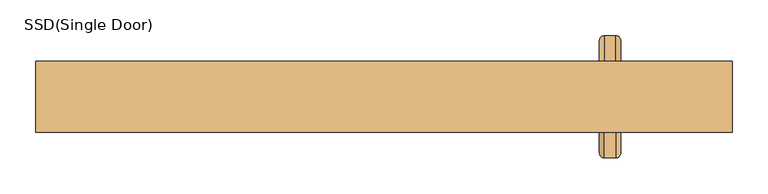
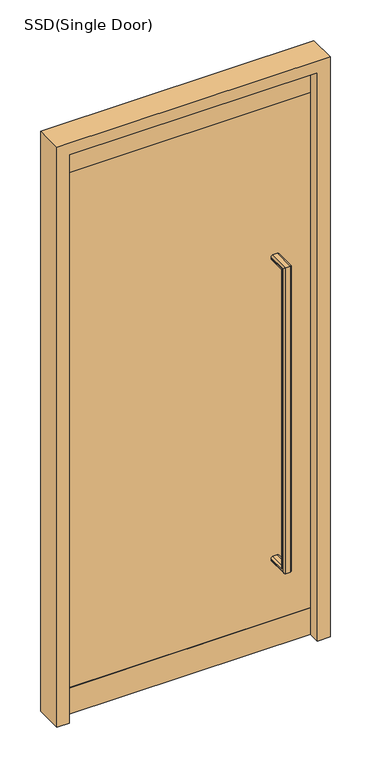
"""IFC4 building model written with IfcOpenShell, lengths in millimetres: door geometry, SSD(Single Door) : H_DR_AR B12_Door_Single_Glass_W1000xH2200_SSD-1."""

from ifc_helpers import new_model, si_unit, frame, origin, origin_with_axes, place, context, project, spatial, polyline, circle_curve, ellipse_curve, outline, extrude, source, transform, mapped, element, save
from ifc_brep_helpers import plane_surface, cylinder_surface, advanced_brep


def ssd_single_door_b9475c77(model_context):
    return source(origin(), model_context, "Body", "SolidModel", [
        extrude(outline(polyline([(0.0, -490.0), (0.0, -445.0), (2155.0, -445.0), (2155.0, 445.0), (0.0, 445.0), (0.0, 490.0), (2200.0, 490.0), (2200.0, -490.0), (0.0, -490.0)])), frame((0.0, -7.0, 0.0), z_axis=(0.0, 1.0, 0.0), x_axis=(0.0, 0.0, 1.0)), (0.0, 0.0, 1.0), 100.0),
        advanced_brep(
        [(310.0, 37.0, 1485.0), (326.0, 37.0, 1485.0), (333.0, 37.0, 1478.0), (333.0, 37.0, 1475.0), (326.0, 37.0, 1468.0), (310.0, 37.0, 1468.0), (303.0, 37.0, 1475.0), (303.0, 37.0, 1478.0), (310.0, 37.0, 325.0), (303.0, 37.0, 332.0), (303.0, 37.0, 335.0), (310.0, 37.0, 342.0), (326.0, 37.0, 342.0), (333.0, 37.0, 335.0), (333.0, 37.0, 332.0), (326.0, 37.0, 325.0), (310.0, -43.0, 1485.0), (326.0, -43.0, 1485.0), (333.0, -36.0, 1478.0), (333.0, -36.0, 332.0), (333.0, -33.0, 335.0), (333.0, -33.0, 1475.0), (326.0, -26.0, 1468.0), (310.0, -26.0, 1468.0), (303.0, -33.0, 1475.0), (303.0, -33.0, 335.0), (303.0, -36.0, 332.0), (303.0, -36.0, 1478.0), (310.0, -43.0, 325.0), (326.0, -43.0, 325.0), (326.0, -26.0, 342.0), (310.0, -26.0, 342.0)],
        [
            (0, 1),
            (1, 2, circle_curve(frame((326.0, 37.0, 1478.0), z_axis=(0.0, 1.0, 0.0), x_axis=(0.0, 0.0, -1.0)), 7.0)),
            (2, 3),
            (3, 4, circle_curve(frame((326.0, 37.0, 1475.0), z_axis=(0.0, 1.0, 0.0), x_axis=(0.0, 0.0, -1.0)), 7.0)),
            (4, 5),
            (5, 6, circle_curve(frame((310.0, 37.0, 1475.0), z_axis=(0.0, 1.0, 0.0), x_axis=(0.0, 0.0, -1.0)), 7.0)),
            (6, 7),
            (7, 0, circle_curve(frame((310.0, 37.0, 1478.0), z_axis=(0.0, 1.0, 0.0), x_axis=(0.0, 0.0, -1.0)), 7.0)),
            (8, 9, circle_curve(frame((310.0, 37.0, 332.0), z_axis=(0.0, 1.0, 0.0), x_axis=(0.0, 0.0, 1.0)), 7.0)),
            (9, 10),
            (10, 11, circle_curve(frame((310.0, 37.0, 335.0), z_axis=(0.0, 1.0, 0.0), x_axis=(0.0, 0.0, 1.0)), 7.0)),
            (11, 12),
            (12, 13, circle_curve(frame((326.0, 37.0, 335.0), z_axis=(0.0, 1.0, 0.0), x_axis=(0.0, 0.0, 1.0)), 7.0)),
            (13, 14),
            (14, 15, circle_curve(frame((326.0, 37.0, 332.0), z_axis=(0.0, 1.0, 0.0), x_axis=(0.0, 0.0, 1.0)), 7.0)),
            (15, 8),
            (0, 16),
            (16, 17),
            (17, 1),
            (17, 18, ellipse_curve(frame((326.0, -36.0, 1478.0), z_axis=(0.0, 0.7071067811865475, 0.7071067811865475), x_axis=(0.0, 0.7071067811865476, -0.7071067811865474)), 9.8994949, 7.0)),
            (18, 2),
            (18, 19),
            (19, 14),
            (13, 20),
            (20, 21),
            (21, 3),
            (21, 22, ellipse_curve(frame((326.0, -33.0, 1475.0), z_axis=(0.0, 0.7071067811865475, 0.7071067811865475), x_axis=(0.0, 0.7071067811865476, -0.7071067811865474)), 9.8994949, 7.0)),
            (22, 4),
            (22, 23),
            (23, 5),
            (23, 24, ellipse_curve(frame((310.0, -33.0, 1475.0), z_axis=(0.0, 0.7071067811865475, 0.7071067811865475), x_axis=(0.0, 0.7071067811865476, -0.7071067811865474)), 9.8994949, 7.0)),
            (24, 6),
            (24, 25),
            (25, 10),
            (9, 26),
            (26, 27),
            (27, 7),
            (27, 16, ellipse_curve(frame((310.0, -36.0, 1478.0), z_axis=(0.0, 0.7071067811865475, 0.7071067811865475), x_axis=(0.0, 0.7071067811865476, -0.7071067811865474)), 9.8994949, 7.0)),
            (16, 28),
            (28, 29),
            (29, 17),
            (29, 19, ellipse_curve(frame((326.0, -36.0, 332.0), z_axis=(0.0, -0.7071067811865475, 0.7071067811865475), x_axis=(0.0, 0.7071067811865474, 0.7071067811865476)), 9.8994949, 7.0)),
            (20, 30, ellipse_curve(frame((326.0, -33.0, 335.0), z_axis=(0.0, -0.7071067811865475, 0.7071067811865475), x_axis=(0.0, 0.7071067811865474, 0.7071067811865476)), 9.8994949, 7.0)),
            (30, 22),
            (30, 31),
            (31, 23),
            (31, 25, ellipse_curve(frame((310.0, -33.0, 335.0), z_axis=(0.0, -0.7071067811865475, 0.7071067811865475), x_axis=(0.0, 0.7071067811865474, 0.7071067811865476)), 9.8994949, 7.0)),
            (26, 28, ellipse_curve(frame((310.0, -36.0, 332.0), z_axis=(0.0, -0.7071067811865475, 0.7071067811865475), x_axis=(0.0, 0.7071067811865474, 0.7071067811865476)), 9.8994949, 7.0)),
            (28, 8),
            (15, 29),
            (12, 30),
            (11, 31),
        ],
        [
            plane_surface(frame((0.0, 37.0, 1485.0), z_axis=(0.0, 1.0, 0.0), x_axis=(1.0, 0.0, 0.0))),
            plane_surface(frame((0.0, 37.0, 325.0), z_axis=(0.0, 1.0, 0.0), x_axis=(1.0, 0.0, 0.0))),
            plane_surface(frame((310.0, 37.0, 1485.0), z_axis=(0.0, 0.0, 1.0), x_axis=(0.0, -1.0, 0.0))),
            cylinder_surface(frame((326.0, 37.0, 1478.0), z_axis=(0.0, 1.0, 0.0), x_axis=(0.0, 0.0, -1.0)), 7.0),
            plane_surface(frame((333.0, 37.0, 1478.0), z_axis=(1.0, 0.0, 0.0), x_axis=(0.0, -1.0, 0.0))),
            cylinder_surface(frame((326.0, 37.0, 1475.0), z_axis=(0.0, 1.0, 0.0), x_axis=(0.0, 0.0, -1.0)), 7.0),
            plane_surface(frame((326.0, 37.0, 1468.0), z_axis=(0.0, 0.0, -1.0), x_axis=(0.0, -1.0, 0.0))),
            cylinder_surface(frame((310.0, 37.0, 1475.0), z_axis=(0.0, 1.0, 0.0), x_axis=(0.0, 0.0, -1.0)), 7.0),
            plane_surface(frame((303.0, 37.0, 1475.0), z_axis=(-1.0, 0.0, 0.0), x_axis=(0.0, -1.0, 0.0))),
            cylinder_surface(frame((310.0, 37.0, 1478.0), z_axis=(0.0, 1.0, 0.0), x_axis=(0.0, 0.0, -1.0)), 7.0),
            plane_surface(frame((310.0, -43.0, 1485.0), z_axis=(0.0, -1.0, 0.0), x_axis=(0.0, 0.0, -1.0))),
            cylinder_surface(frame((326.0, -36.0, 1485.0), z_axis=(0.0, 0.0, 1.0), x_axis=(0.0, 1.0, 0.0)), 7.0),
            cylinder_surface(frame((326.0, -33.0, 1485.0), z_axis=(0.0, 0.0, 1.0), x_axis=(0.0, 1.0, 0.0)), 7.0),
            plane_surface(frame((326.0, -26.0, 1468.0), z_axis=(0.0, 1.0, 0.0), x_axis=(0.0, 0.0, -1.0))),
            cylinder_surface(frame((310.0, -33.0, 1485.0), z_axis=(0.0, 0.0, 1.0), x_axis=(0.0, 1.0, 0.0)), 7.0),
            cylinder_surface(frame((310.0, -36.0, 1485.0), z_axis=(0.0, 0.0, 1.0), x_axis=(0.0, 1.0, 0.0)), 7.0),
            plane_surface(frame((310.0, -43.0, 325.0), z_axis=(0.0, 0.0, -1.0), x_axis=(0.0, 1.0, 0.0))),
            cylinder_surface(frame((326.0, -43.0, 332.0), z_axis=(0.0, -1.0, 0.0), x_axis=(0.0, 0.0, 1.0)), 7.0),
            cylinder_surface(frame((326.0, -43.0, 335.0), z_axis=(0.0, -1.0, 0.0), x_axis=(0.0, 0.0, 1.0)), 7.0),
            plane_surface(frame((326.0, -26.0, 342.0), z_axis=(0.0, 0.0, 1.0), x_axis=(0.0, 1.0, 0.0))),
            cylinder_surface(frame((310.0, -43.0, 335.0), z_axis=(0.0, -1.0, 0.0), x_axis=(0.0, 0.0, 1.0)), 7.0),
            cylinder_surface(frame((310.0, -43.0, 332.0), z_axis=(0.0, -1.0, 0.0), x_axis=(0.0, 0.0, 1.0)), 7.0),
        ],
        [
            (0, [[1, 2, 3, 4, 5, 6, 7, 8]]),
            (1, [[9, 10, 11, 12, 13, 14, 15, 16]]),
            (2, [[-1, 17, 18, 19]]),
            (3, [[-2, -19, 20, 21]]),
            (4, [[-3, -21, 22, 23, -14, 24, 25, 26]]),
            (5, [[-4, -26, 27, 28]]),
            (6, [[-5, -28, 29, 30]]),
            (7, [[-6, -30, 31, 32]]),
            (8, [[-7, -32, 33, 34, -10, 35, 36, 37]]),
            (9, [[-8, -37, 38, -17]]),
            (10, [[-18, 39, 40, 41]]),
            (11, [[-20, -41, 42, -22]]),
            (12, [[-27, -25, 43, 44]]),
            (13, [[-29, -44, 45, 46]]),
            (14, [[-31, -46, 47, -33]]),
            (15, [[-38, -36, 48, -39]]),
            (16, [[-40, 49, -16, 50]]),
            (17, [[-42, -50, -15, -23]]),
            (18, [[-43, -24, -13, 51]]),
            (19, [[-45, -51, -12, 52]]),
            (20, [[-47, -52, -11, -34]]),
            (21, [[-48, -35, -9, -49]]),
        ],
    ),
        advanced_brep(
        [(310.0, 49.0, 1485.0), (303.0, 49.0, 1478.0), (303.0, 49.0, 1475.0), (310.0, 49.0, 1468.0), (326.0, 49.0, 1468.0), (333.0, 49.0, 1475.0), (333.0, 49.0, 1478.0), (326.0, 49.0, 1485.0), (310.0, 49.0, 325.0), (326.0, 49.0, 325.0), (333.0, 49.0, 332.0), (333.0, 49.0, 335.0), (326.0, 49.0, 342.0), (310.0, 49.0, 342.0), (303.0, 49.0, 335.0), (303.0, 49.0, 332.0), (310.0, 129.0, 1485.0), (303.0, 122.0, 1478.0), (303.0, 122.0, 332.0), (303.0, 119.0, 335.0), (303.0, 119.0, 1475.0), (310.0, 112.0, 1468.0), (326.0, 112.0, 1468.0), (333.0, 119.0, 1475.0), (333.0, 119.0, 335.0), (333.0, 122.0, 332.0), (333.0, 122.0, 1478.0), (326.0, 129.0, 1485.0), (310.0, 129.0, 325.0), (310.0, 112.0, 342.0), (326.0, 112.0, 342.0), (326.0, 129.0, 325.0)],
        [
            (0, 1, circle_curve(frame((310.0, 49.0, 1478.0), z_axis=(0.0, -1.0, 0.0), x_axis=(0.0, 0.0, 1.0)), 7.0)),
            (1, 2),
            (2, 3, circle_curve(frame((310.0, 49.0, 1475.0), z_axis=(0.0, -1.0, 0.0), x_axis=(0.0, 0.0, 1.0)), 7.0)),
            (3, 4),
            (4, 5, circle_curve(frame((326.0, 49.0, 1475.0), z_axis=(0.0, -1.0, 0.0), x_axis=(0.0, 0.0, 1.0)), 7.0)),
            (5, 6),
            (6, 7, circle_curve(frame((326.0, 49.0, 1478.0), z_axis=(0.0, -1.0, 0.0), x_axis=(0.0, 0.0, 1.0)), 7.0)),
            (7, 0),
            (8, 9),
            (9, 10, circle_curve(frame((326.0, 49.0, 332.0), z_axis=(0.0, -1.0, 0.0), x_axis=(0.0, 0.0, -1.0)), 7.0)),
            (10, 11),
            (11, 12, circle_curve(frame((326.0, 49.0, 335.0), z_axis=(0.0, -1.0, 0.0), x_axis=(0.0, 0.0, -1.0)), 7.0)),
            (12, 13),
            (13, 14, circle_curve(frame((310.0, 49.0, 335.0), z_axis=(0.0, -1.0, 0.0), x_axis=(0.0, 0.0, -1.0)), 7.0)),
            (14, 15),
            (15, 8, circle_curve(frame((310.0, 49.0, 332.0), z_axis=(0.0, -1.0, 0.0), x_axis=(0.0, 0.0, -1.0)), 7.0)),
            (0, 16),
            (16, 17, ellipse_curve(frame((310.0, 122.0, 1478.0), z_axis=(0.0, -0.7071067811865475, 0.7071067811865475), x_axis=(0.0, -0.7071067811865476, -0.7071067811865474)), 9.8994949, 7.0)),
            (17, 1),
            (17, 18),
            (18, 15),
            (14, 19),
            (19, 20),
            (20, 2),
            (20, 21, ellipse_curve(frame((310.0, 119.0, 1475.0), z_axis=(0.0, -0.7071067811865475, 0.7071067811865475), x_axis=(0.0, -0.7071067811865476, -0.7071067811865474)), 9.8994949, 7.0)),
            (21, 3),
            (21, 22),
            (22, 4),
            (22, 23, ellipse_curve(frame((326.0, 119.0, 1475.0), z_axis=(0.0, -0.7071067811865475, 0.7071067811865475), x_axis=(0.0, -0.7071067811865476, -0.7071067811865474)), 9.8994949, 7.0)),
            (23, 5),
            (23, 24),
            (24, 11),
            (10, 25),
            (25, 26),
            (26, 6),
            (26, 27, ellipse_curve(frame((326.0, 122.0, 1478.0), z_axis=(0.0, -0.7071067811865475, 0.7071067811865475), x_axis=(0.0, -0.7071067811865476, -0.7071067811865474)), 9.8994949, 7.0)),
            (27, 7),
            (27, 16),
            (16, 28),
            (28, 18, ellipse_curve(frame((310.0, 122.0, 332.0), z_axis=(0.0, 0.7071067811865475, 0.7071067811865475), x_axis=(0.0, -0.7071067811865474, 0.7071067811865476)), 9.8994949, 7.0)),
            (19, 29, ellipse_curve(frame((310.0, 119.0, 335.0), z_axis=(0.0, 0.7071067811865475, 0.7071067811865475), x_axis=(0.0, -0.7071067811865474, 0.7071067811865476)), 9.8994949, 7.0)),
            (29, 21),
            (29, 30),
            (30, 22),
            (30, 24, ellipse_curve(frame((326.0, 119.0, 335.0), z_axis=(0.0, 0.7071067811865475, 0.7071067811865475), x_axis=(0.0, -0.7071067811865474, 0.7071067811865476)), 9.8994949, 7.0)),
            (25, 31, ellipse_curve(frame((326.0, 122.0, 332.0), z_axis=(0.0, 0.7071067811865475, 0.7071067811865475), x_axis=(0.0, -0.7071067811865474, 0.7071067811865476)), 9.8994949, 7.0)),
            (31, 27),
            (31, 28),
            (28, 8),
            (13, 29),
            (12, 30),
            (9, 31),
        ],
        [
            plane_surface(frame((0.0, 49.0, 1485.0), z_axis=(0.0, -1.0, 0.0), x_axis=(1.0, 0.0, 0.0))),
            plane_surface(frame((0.0, 49.0, 325.0), z_axis=(0.0, -1.0, 0.0), x_axis=(1.0, 0.0, 0.0))),
            cylinder_surface(frame((310.0, 49.0, 1478.0), z_axis=(0.0, -1.0, 0.0), x_axis=(0.0, 0.0, 1.0)), 7.0),
            plane_surface(frame((303.0, 49.0, 1478.0), z_axis=(-1.0, 0.0, 0.0), x_axis=(0.0, 1.0, 0.0))),
            cylinder_surface(frame((310.0, 49.0, 1475.0), z_axis=(0.0, -1.0, 0.0), x_axis=(0.0, 0.0, 1.0)), 7.0),
            plane_surface(frame((310.0, 49.0, 1468.0), z_axis=(0.0, 0.0, -1.0), x_axis=(0.0, 1.0, 0.0))),
            cylinder_surface(frame((326.0, 49.0, 1475.0), z_axis=(0.0, -1.0, 0.0), x_axis=(0.0, 0.0, 1.0)), 7.0),
            plane_surface(frame((333.0, 49.0, 1475.0), z_axis=(1.0, 0.0, 0.0), x_axis=(0.0, 1.0, 0.0))),
            cylinder_surface(frame((326.0, 49.0, 1478.0), z_axis=(0.0, -1.0, 0.0), x_axis=(0.0, 0.0, 1.0)), 7.0),
            plane_surface(frame((326.0, 49.0, 1485.0), z_axis=(0.0, 0.0, 1.0), x_axis=(0.0, 1.0, 0.0))),
            cylinder_surface(frame((310.0, 122.0, 1485.0), z_axis=(0.0, 0.0, 1.0), x_axis=(0.0, 1.0, 0.0)), 7.0),
            cylinder_surface(frame((310.0, 119.0, 1485.0), z_axis=(0.0, 0.0, 1.0), x_axis=(0.0, 1.0, 0.0)), 7.0),
            plane_surface(frame((310.0, 112.0, 1468.0), z_axis=(0.0, -1.0, 0.0), x_axis=(0.0, 0.0, -1.0))),
            cylinder_surface(frame((326.0, 119.0, 1485.0), z_axis=(0.0, 0.0, 1.0), x_axis=(0.0, 1.0, 0.0)), 7.0),
            cylinder_surface(frame((326.0, 122.0, 1485.0), z_axis=(0.0, 0.0, 1.0), x_axis=(0.0, 1.0, 0.0)), 7.0),
            plane_surface(frame((326.0, 129.0, 1485.0), z_axis=(0.0, 1.0, 0.0), x_axis=(0.0, 0.0, -1.0))),
            cylinder_surface(frame((310.0, 129.0, 332.0), z_axis=(0.0, 1.0, 0.0), x_axis=(0.0, 0.0, -1.0)), 7.0),
            cylinder_surface(frame((310.0, 129.0, 335.0), z_axis=(0.0, 1.0, 0.0), x_axis=(0.0, 0.0, -1.0)), 7.0),
            plane_surface(frame((310.0, 112.0, 342.0), z_axis=(0.0, 0.0, 1.0), x_axis=(0.0, -1.0, 0.0))),
            cylinder_surface(frame((326.0, 129.0, 335.0), z_axis=(0.0, 1.0, 0.0), x_axis=(0.0, 0.0, -1.0)), 7.0),
            cylinder_surface(frame((326.0, 129.0, 332.0), z_axis=(0.0, 1.0, 0.0), x_axis=(0.0, 0.0, -1.0)), 7.0),
            plane_surface(frame((326.0, 129.0, 325.0), z_axis=(0.0, 0.0, -1.0), x_axis=(0.0, -1.0, 0.0))),
        ],
        [
            (0, [[1, 2, 3, 4, 5, 6, 7, 8]]),
            (1, [[9, 10, 11, 12, 13, 14, 15, 16]]),
            (2, [[-1, 17, 18, 19]]),
            (3, [[-2, -19, 20, 21, -15, 22, 23, 24]]),
            (4, [[-3, -24, 25, 26]]),
            (5, [[-4, -26, 27, 28]]),
            (6, [[-5, -28, 29, 30]]),
            (7, [[-6, -30, 31, 32, -11, 33, 34, 35]]),
            (8, [[-7, -35, 36, 37]]),
            (9, [[-8, -37, 38, -17]]),
            (10, [[-18, 39, 40, -20]]),
            (11, [[-25, -23, 41, 42]]),
            (12, [[-27, -42, 43, 44]]),
            (13, [[-29, -44, 45, -31]]),
            (14, [[-36, -34, 46, 47]]),
            (15, [[-38, -47, 48, -39]]),
            (16, [[-40, 49, -16, -21]]),
            (17, [[-41, -22, -14, 50]]),
            (18, [[-43, -50, -13, 51]]),
            (19, [[-45, -51, -12, -32]]),
            (20, [[-46, -33, -10, 52]]),
            (21, [[-48, -52, -9, -49]]),
        ],
    ),
        extrude(outline(polyline([(445.0, 37.0), (-445.0, 37.0), (-445.0, 49.0), (445.0, 49.0), (445.0, 37.0)])), frame((0.0, 0.0, 100.0), z_axis=(0.0, 0.0, 1.0), x_axis=(1.0, 0.0, 0.0)), (0.0, 0.0, 1.0), 1955.0),
        extrude(outline(polyline([(445.0, 35.0), (-445.0, 35.0), (-445.0, 51.0), (445.0, 51.0), (445.0, 35.0)])), frame((0.0, 0.0, 2055.0), z_axis=(0.0, 0.0, 1.0), x_axis=(1.0, 0.0, 0.0)), (0.0, 0.0, 1.0), 100.0),
        extrude(outline(polyline([(445.0, 35.0), (-445.0, 35.0), (-445.0, 51.0), (445.0, 51.0), (445.0, 35.0)])), origin_with_axes(), (0.0, 0.0, 1.0), 100.0),
    ])


if __name__ == "__main__":
    model = new_model("IFC4")
    model_context = context("Model", 3, world=origin())
    ifc_project = project(units=[si_unit("LENGTHUNIT", "METRE", prefix="MILLI")], contexts=[model_context])
    site = spatial("IfcSite", under=ifc_project)
    building = spatial("IfcBuilding", under=site)
    placement = place(None, origin())
    ssd_single_door_shape = ssd_single_door_b9475c77(model_context)
    element("IfcDoor", 1, ObjectType="SSD(Single Door) : H_DR_AR B12_Door_Single_Glass_W1000xH2200_SSD-1", at=placement, inside=building, context=model_context, shape_type="MappedRepresentation", body=[
        mapped(ssd_single_door_shape, transform((0.0, 0.0, 0.0), x_axis=(1.0, 0.0, 0.0), y_axis=(0.0, 1.0, 0.0), z_axis=(0.0, 0.0, 1.0))),
    ])
    save(model, "model.ifc")

# Revit data of these elements
# Type "SSD(Single Door) : H_DR_AR B12_Door_Single_Glass_W1000xH2200_SSD-1"
#   Type Mark = "452"
#   Type Comments = "SSD"
#   Analytic Construction = "<None>"
#   Thickness = 45 mm
#   Plan Door Swing2 = 890 mm
#   Plan Door Swing = 1780 mm
#   Glass Thk = 12 mm
#   Frame THK = 100 mm
#   Frame Projection Ext. = 25 mm
#   Frame Projection Int. = 25 mm
#   Frame Width = 75 mm
#   Height = 2200 mm
#   Width = 980 mm
#   Center Door [instance default] = 100 mm
#   Define Thermal Properties by = 1
#   Function = (empty or 0)
#   Wall Closure = (empty or 0)
# Element 1 (IfcDoor, "SSD(Single Door) : H_DR_AR B12_Door_Single_Glass_W1000xH2200_SSD-1")
#   Center Door = 43 mm
#   Materials on its faces: "Stainless Steel", "Glass"
# Materials
#   "Stainless Steel": class "Metal", colour RGB 189 187 185, transparency 0, Description = "Stainless Steel 18/8", Cost = 0
#   "Glass": class "Glass", colour RGB 218 227 224, transparency 0.85, Description = "Soda Lime Glass", Cost = 0
